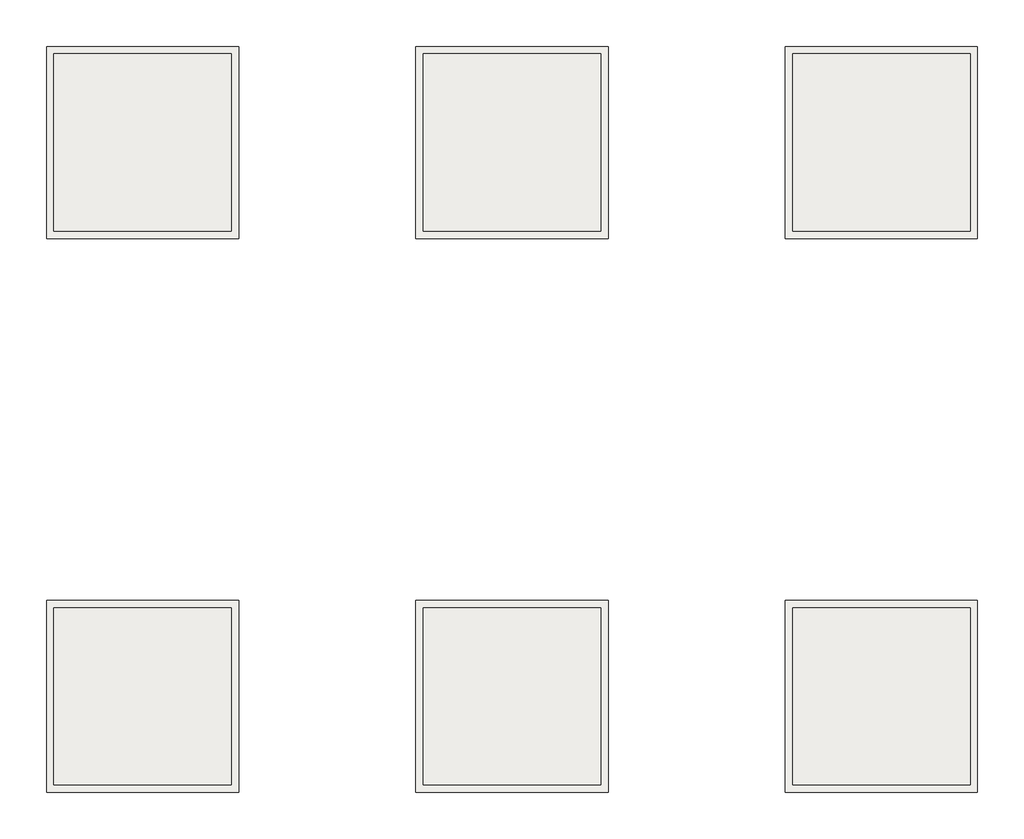
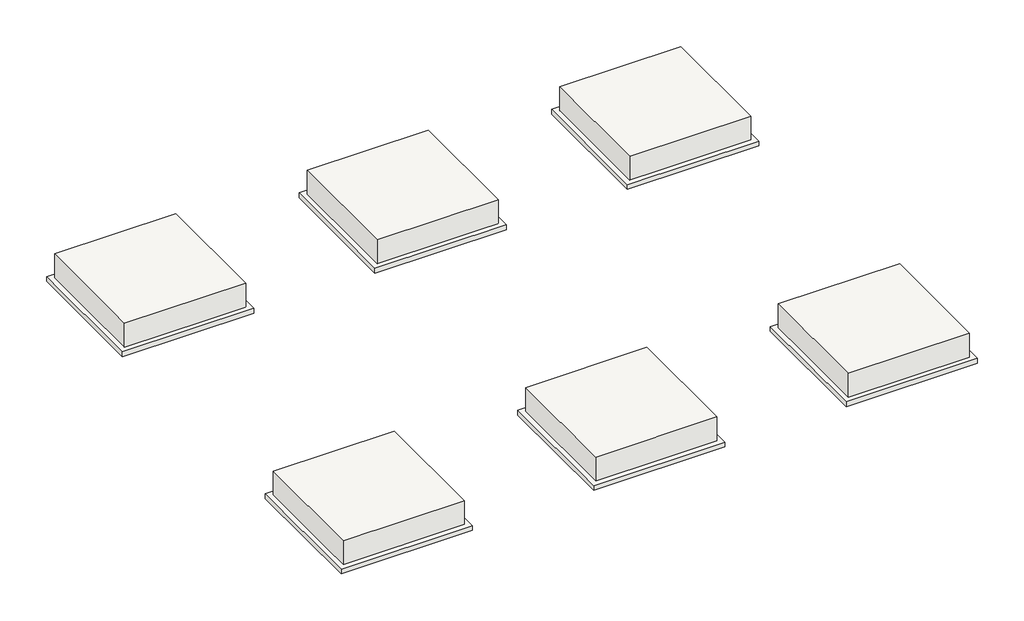
# Not in any storey: 12 slabs.
"""IFC4 building model written with IfcOpenShell, lengths in millimetres."""

import ifcopenshell
import ifcopenshell.guid

model = None  # the IFC model being written
_history = None  # IfcOwnerHistory: only IFC2X3 demands one
_inside = {}  # id of a spatial element -> (the spatial element, [elements in it])
_under = {}  # id of a project, library or spatial element -> (it, [spatial elements below it])
_declared = {}  # id of a project -> (the project, [libraries it declares])
_typed = {}  # id of a type object -> (the type object, [elements of that type])
_made_of = {}  # id of a material, layer set ... -> (it, [elements and type objects made of it])


def new_model(schema):
    """Start an empty IFC model of exactly this schema.

    Asked for "IFC4X3", IfcOpenShell would pick the latest addendum, in which some entities
    have other attributes; the version numbers below select the first issue.
    IFC2X3 requires an IfcOwnerHistory on every rooted entity: one is made here for all.
    """
    global model, _history
    if schema == "IFC4X3":
        model = ifcopenshell.file(schema_version=(4, 3, 0, 0))
    else:
        model = ifcopenshell.file(schema=schema)
    _inside.clear()
    _under.clear()
    _declared.clear()
    _typed.clear()
    _made_of.clear()
    _history = None
    if model.schema == "IFC2X3":
        org = make("IfcOrganization", Name="unknown")
        user = make(
            "IfcPersonAndOrganization",
            ThePerson=make("IfcPerson", FamilyName="unknown"),
            TheOrganization=org,
        )
        app = make(
            "IfcApplication",
            ApplicationDeveloper=org,
            Version="unknown",
            ApplicationFullName="unknown",
            ApplicationIdentifier="unknown",
        )
        _history = make(
            "IfcOwnerHistory",
            OwningUser=user,
            OwningApplication=app,
            ChangeAction="ADDED",
            CreationDate=0,
        )
    return model


def make(cls, **values):
    """One entity of the class cls with the attributes given. An attribute that is None is left unset."""
    return model.create_entity(
        cls, **{name: value for name, value in values.items() if value is not None}
    )


def rooted(cls, **values):
    """An entity with a GlobalId (a new one), such as an element, a storey or a relation."""
    return make(cls, GlobalId=ifcopenshell.guid.new(), OwnerHistory=_history, **values)


def si_unit(unit_type, name, prefix=None):
    """IfcSIUnit, for example si_unit("LENGTHUNIT", "METRE", prefix="MILLI")."""
    return make("IfcSIUnit", UnitType=unit_type, Prefix=prefix, Name=name)


def assignment(units):
    """IfcUnitAssignment: the units of a project."""
    return None if units is None else make("IfcUnitAssignment", Units=units)


def point(xyz):
    """IfcCartesianPoint."""
    return None if xyz is None else make("IfcCartesianPoint", Coordinates=xyz)


def direction(xyz):
    """IfcDirection."""
    return None if xyz is None else make("IfcDirection", DirectionRatios=xyz)


def frame(location, z_axis=None, x_axis=None):
    """IfcAxis2Placement3D, a coordinate frame: its origin and axes. An axis left out is left unset."""
    return make(
        "IfcAxis2Placement3D",
        Location=point(location),
        Axis=direction(z_axis),
        RefDirection=direction(x_axis),
    )


def origin():
    """The frame at (0, 0, 0) with its axes left unset."""
    return frame((0.0, 0.0, 0.0))


def place(relative_to, where):
    """IfcLocalPlacement: puts the frame where relative to a parent placement (None: the world)."""
    return make(
        "IfcLocalPlacement", PlacementRelTo=relative_to, RelativePlacement=where
    )


def context(
    kind, dimensions, precision=None, world=None, true_north=None, identifier=None
):
    """IfcGeometricRepresentationContext, for example the 3D "Model" context."""
    return make(
        "IfcGeometricRepresentationContext",
        ContextIdentifier=identifier,
        ContextType=kind,
        CoordinateSpaceDimension=dimensions,
        Precision=precision,
        WorldCoordinateSystem=world,
        TrueNorth=true_north,
    )


def project(units=None, contexts=None):
    """IfcProject with its units and contexts."""
    return rooted(
        "IfcProject",
        Name="project",
        RepresentationContexts=contexts,
        UnitsInContext=assignment(units),
    )


def spatial(cls, under=None, at=None, **own):
    """A site, building, storey or space (cls), placed at a placement, below another one or the project."""
    s = rooted(cls, ObjectPlacement=at, **own)
    if under is not None:
        _under.setdefault(under.id(), (under, []))[1].append(s)
    return s


def polyline(points):
    """IfcPolyline through the points."""
    return make("IfcPolyline", Points=[point(p) for p in points])


def outline(outer, holes=None, kind="AREA"):
    """IfcArbitraryClosedProfileDef: a profile drawn as a closed curve; with holes, ...WithVoids."""
    if holes is None:
        return make("IfcArbitraryClosedProfileDef", ProfileType=kind, OuterCurve=outer)
    return make(
        "IfcArbitraryProfileDefWithVoids",
        ProfileType=kind,
        OuterCurve=outer,
        InnerCurves=holes,
    )


def extrude(swept, where, along, depth):
    """IfcExtrudedAreaSolid: the profile swept, set in the frame where, extruded along a direction by depth."""
    return make(
        "IfcExtrudedAreaSolid",
        SweptArea=swept,
        Position=where,
        ExtrudedDirection=direction(along),
        Depth=depth,
    )


def shape(context_of_items, identifier, shape_type, items):
    """IfcShapeRepresentation: the items that make up one representation, for example the "Body"."""
    return make(
        "IfcShapeRepresentation",
        ContextOfItems=context_of_items,
        RepresentationIdentifier=identifier,
        RepresentationType=shape_type,
        Items=items,
    )


def made_of(thing, what):
    """Note that an element or type object is made of a material, layer set ...; save() writes the relation."""
    if what is not None:
        _made_of.setdefault(what.id(), (what, []))[1].append(thing)
    return thing


def element(
    cls,
    number,
    at=None,
    inside=None,
    cuts=None,
    type_object=None,
    material=None,
    context=None,
    identifier="Body",
    shape_type=None,
    held_by="IfcProductDefinitionShape",
    body=None,
    shapes=None,
    **own,
):
    """One element of the class cls, such as IfcWall. Its Tag is "e" and its number.

    at: its placement. inside: the storey or other place that contains it. cuts: it is an
    opening in that element (IfcRelVoidsElement). A single representation is given by context,
    identifier, shape_type and body (its items); several are given by shapes. held_by: the class
    of the entity that holds the representations. save() writes the other relations.
    """
    e = rooted(cls, Tag="e%d" % number, ObjectPlacement=at, **own)
    if body is not None:
        shapes = [shape(context, identifier, shape_type, body)]
    if shapes is not None:
        e.Representation = make(held_by, Representations=shapes)
    if inside is not None:
        _inside.setdefault(inside.id(), (inside, []))[1].append(e)
    if cuts is not None:
        rooted(
            "IfcRelVoidsElement", RelatingBuildingElement=cuts, RelatedOpeningElement=e
        )
    if type_object is not None:
        _typed.setdefault(type_object.id(), (type_object, []))[1].append(e)
    return made_of(e, material)


def aggregate(whole, parts):
    """IfcRelAggregates: a whole, such as a stair, and the parts it consists of."""
    return rooted("IfcRelAggregates", RelatingObject=whole, RelatedObjects=parts)


def save(model, path):
    """Write the relations noted so far, then the file.

    IfcRelAggregates (storeys below a building ...), IfcRelContainedInSpatialStructure (elements
    in a storey), IfcRelDefinesByType, IfcRelAssociatesMaterial and IfcRelDeclares: one each for
    every whole, place, type object, material and project.
    """
    for whole, parts in _under.values():
        aggregate(whole, parts)
    for where, things in _inside.values():
        rooted(
            "IfcRelContainedInSpatialStructure",
            RelatedElements=things,
            RelatingStructure=where,
        )
    for kind, things in _typed.values():
        rooted("IfcRelDefinesByType", RelatedObjects=things, RelatingType=kind)
    for what, things in _made_of.values():
        rooted("IfcRelAssociatesMaterial", RelatedObjects=things, RelatingMaterial=what)
    for by, libraries in _declared.values():
        rooted("IfcRelDeclares", RelatingContext=by, RelatedDefinitions=libraries)
    model.write(path)


model = new_model("IFC4")

# Units and contexts
model_context = context("Model", 3, world=origin())
ifc_project = project(units=[si_unit("LENGTHUNIT", "METRE", prefix="MILLI")], contexts=[model_context])

# Site, building
site = spatial("IfcSite", under=ifc_project)
building = spatial("IfcBuilding", under=site)

# Slabs
placement = place(None, origin())
element("IfcSlab", 1, ObjectType="H_SF_ACF_Lean_T100", at=placement, inside=building, context=model_context, shape_type="SweptSolid", body=[
    extrude(outline(polyline([(-1300.0, 22299.5208589), (1300.0, 22299.5208589), (1300.0, 19699.5208589), (-1300.0, 19699.5208589), (-1300.0, 22299.5208589)])), frame((0.0, 0.0, -1600.0), z_axis=(0.0, 0.0, 1.0), x_axis=(1.0, 0.0, 0.0)), (0.0, 0.0, 1.0), 100.0),
])
element("IfcSlab", 2, ObjectType="H_SF_ACF_Lean_T100", at=placement, inside=building, context=model_context, shape_type="SweptSolid", body=[
    extrude(outline(polyline([(-1300.0, 14799.5208589), (1300.0, 14799.5208589), (1300.0, 12199.5208589), (-1300.0, 12199.5208589), (-1300.0, 14799.5208589)])), frame((0.0, 0.0, -1600.0), z_axis=(0.0, 0.0, 1.0), x_axis=(1.0, 0.0, 0.0)), (0.0, 0.0, 1.0), 100.0),
])
element("IfcSlab", 3, ObjectType="H_SF_ACF_Lean_T100", at=placement, inside=building, context=model_context, shape_type="SweptSolid", body=[
    extrude(outline(polyline([(3700.0, 22299.5208589), (6300.0, 22299.5208589), (6300.0, 19699.5208589), (3700.0, 19699.5208589), (3700.0, 22299.5208589)])), frame((0.0, 0.0, -1600.0), z_axis=(0.0, 0.0, 1.0), x_axis=(1.0, 0.0, 0.0)), (0.0, 0.0, 1.0), 100.0),
])
element("IfcSlab", 4, ObjectType="H_SF_ACF_Lean_T100", at=placement, inside=building, context=model_context, shape_type="SweptSolid", body=[
    extrude(outline(polyline([(3700.0, 14799.5208589), (6300.0, 14799.5208589), (6300.0, 12199.5208589), (3700.0, 12199.5208589), (3700.0, 14799.5208589)])), frame((0.0, 0.0, -1600.0), z_axis=(0.0, 0.0, 1.0), x_axis=(1.0, 0.0, 0.0)), (0.0, 0.0, 1.0), 100.0),
])
element("IfcSlab", 5, ObjectType="H_SF_ACF_Lean_T100", at=placement, inside=building, context=model_context, shape_type="SweptSolid", body=[
    extrude(outline(polyline([(8700.0, 22299.5208589), (11300.0, 22299.5208589), (11300.0, 19699.5208589), (8700.0, 19699.5208589), (8700.0, 22299.5208589)])), frame((0.0, 0.0, -1600.0), z_axis=(0.0, 0.0, 1.0), x_axis=(1.0, 0.0, 0.0)), (0.0, 0.0, 1.0), 100.0),
])
element("IfcSlab", 6, ObjectType="H_SF_ACF_Lean_T100", at=placement, inside=building, context=model_context, shape_type="SweptSolid", body=[
    extrude(outline(polyline([(8700.0, 14799.5208589), (11300.0, 14799.5208589), (11300.0, 12199.5208589), (8700.0, 12199.5208589), (8700.0, 14799.5208589)])), frame((0.0, 0.0, -1600.0), z_axis=(0.0, 0.0, 1.0), x_axis=(1.0, 0.0, 0.0)), (0.0, 0.0, 1.0), 100.0),
])
element("IfcSlab", 7, ObjectType="Foundation Rectangular (Non-Pile) : H_SF_ACF_W2400xL2400xT500", at=placement, inside=building, context=model_context, shape_type="SweptSolid", body=[
    extrude(outline(polyline([(6200.0, 14699.5208589), (6200.0, 12299.5208589), (3800.0, 12299.5208589), (3800.0, 14699.5208589), (6200.0, 14699.5208589)])), frame((0.0, 0.0, -1500.0), z_axis=(0.0, 0.0, 1.0), x_axis=(1.0, 0.0, 0.0)), (0.0, 0.0, 1.0), 500.0),
])
element("IfcSlab", 8, ObjectType="Foundation Rectangular (Non-Pile) : H_SF_ACF_W2400xL2400xT500", at=placement, inside=building, context=model_context, shape_type="SweptSolid", body=[
    extrude(outline(polyline([(11200.0, 14699.5208589), (11200.0, 12299.5208589), (8800.0, 12299.5208589), (8800.0, 14699.5208589), (11200.0, 14699.5208589)])), frame((0.0, 0.0, -1500.0), z_axis=(0.0, 0.0, 1.0), x_axis=(1.0, 0.0, 0.0)), (0.0, 0.0, 1.0), 500.0),
])
element("IfcSlab", 9, ObjectType="Foundation Rectangular (Non-Pile) : H_SF_ACF_W2400xL2400xT500", at=placement, inside=building, context=model_context, shape_type="SweptSolid", body=[
    extrude(outline(polyline([(11200.0, 22199.5208589), (11200.0, 19799.5208589), (8800.0, 19799.5208589), (8800.0, 22199.5208589), (11200.0, 22199.5208589)])), frame((0.0, 0.0, -1500.0), z_axis=(0.0, 0.0, 1.0), x_axis=(1.0, 0.0, 0.0)), (0.0, 0.0, 1.0), 500.0),
])
element("IfcSlab", 10, ObjectType="Foundation Rectangular (Non-Pile) : H_SF_ACF_W2400xL2400xT500", at=placement, inside=building, context=model_context, shape_type="SweptSolid", body=[
    extrude(outline(polyline([(6200.0, 22199.5208589), (6200.0, 19799.5208589), (3800.0, 19799.5208589), (3800.0, 22199.5208589), (6200.0, 22199.5208589)])), frame((0.0, 0.0, -1500.0), z_axis=(0.0, 0.0, 1.0), x_axis=(1.0, 0.0, 0.0)), (0.0, 0.0, 1.0), 500.0),
])
element("IfcSlab", 11, ObjectType="Foundation Rectangular (Non-Pile) : H_SF_ACF_W2400xL2400xT500", at=placement, inside=building, context=model_context, shape_type="SweptSolid", body=[
    extrude(outline(polyline([(1200.0, 22199.5208589), (1200.0, 19799.5208589), (-1200.0, 19799.5208589), (-1200.0, 22199.5208589), (1200.0, 22199.5208589)])), frame((0.0, 0.0, -1500.0), z_axis=(0.0, 0.0, 1.0), x_axis=(1.0, 0.0, 0.0)), (0.0, 0.0, 1.0), 500.0),
])
element("IfcSlab", 12, ObjectType="Foundation Rectangular (Non-Pile) : H_SF_ACF_W2400xL2400xT500", at=placement, inside=building, context=model_context, shape_type="SweptSolid", body=[
    extrude(outline(polyline([(1200.0, 14699.5208589), (1200.0, 12299.5208589), (-1200.0, 12299.5208589), (-1200.0, 14699.5208589), (1200.0, 14699.5208589)])), frame((0.0, 0.0, -1500.0), z_axis=(0.0, 0.0, 1.0), x_axis=(1.0, 0.0, 0.0)), (0.0, 0.0, 1.0), 500.0),
])

save(model, "model.ifc")

# Revit data of these elements
# Project information
#   Building Name = "MAIN GATE SECURITY BUILDING"
#   Project Status = "Project Status"
#   Client Name = "현대엔지니어링"
#   Project Address = "서울시 종로구 율곡로 75(계동)"
#   Project Name = "Therma Visayas Energy Project"
#   Project Number = "-"
#   BuildingbookInternationalBuildNumber = "ZgA=BAAAAA==2023BgFlAAAAAQoAAAABAQAAAAYBZAAAAAHnBwAABAQAAAABWwIAAAcH0"
# Grids (mm)
#   "A": line (0, 24502.793) -> (0, 11308.625)
#   "B": line (5000, 24502.793) -> (5000, 11308.625)
#   "C": line (10000, 24502.793) -> (10000, 11308.625)
#   "1": line (-3860.098, 13499.521) -> (12441.468, 13499.521)
#   "2": line (-3860.098, 20999.521) -> (12441.468, 20999.521)
# Type "H_SF_ACF_Lean_T100"
#   Type Comments = "구조_콘크리트"
#   Layers, outside or top first: 0.0000 m "A04AR138-00003_Hardener Finish(Powder Type)" (function 100); 0.1000 m "A03AC034-00004_Lean Concrete (including Form work)" (function 1); 0.0000 m "A03AC035-00001_Form Work (3 times in use)_Flat" (function 100); 0.0000 m "A01ZZ012-00001_PE Sheet (Vapor Barrier)_Earth" (function 100)
# Type "Foundation Rectangular (Non-Pile) : H_SF_ACF_W2400xL2400xT500"
#   Top bar = "D25@300"
#   Description = "UG Shallow Foundation"
#   Bottom bar = "D20@300"
#   Width = 2.4000 m
#   Length = 2.4000 m
#   Foundation Thickness = 0.5000 m
#   Structural Material [instance default] = A03AC032-00007_Structural Concrete_Type1_25MPa-30Mpa
#   Assembly Code = ""
# Elements 1, 2, 3, 4, 5, 6 (IfcSlab, "H_SF_ACF_Lean_T100")
#   Comments = ""
#   Height Offset From Level = 0.0000 m
#   built-in parameter 1001954 = 1
#   Phase Created = New Construction
#   Materials on its faces: "A01ZZ012-00001_PE Sheet (Vapor Barrier)_Earth", "A04AR138-00003_Hardener Finish(Powder Type)"
# Elements 7, 8, 9, 10, 11, 12 (IfcSlab, "Foundation Rectangular (Non-Pile) : H_SF_ACF_W2400xL2400xT500")
#   Comments = ""
#   Mark = "F1"
#   Structural Material = A03AC032-00007_Structural Concrete_Type1_25MPa-30Mpa
#   Phase Created = New Construction
#   Materials on its faces: "A03AC032-00007_Structural Concrete_Type1_25MPa-30Mpa"
# Materials
#   "A04AR138-00003_Hardener Finish(Powder Type)": class "Finish", colour RGB 176 176 176, transparency 0, Description = "Hardner", Cost = 0
#   "A03AC034-00004_Lean Concrete (including Form work)": class "Concrete", colour RGB 176 176 176, transparency 0, Description = "Plain Conc.", Cost = 0
#   "A03AC035-00001_Form Work (3 times in use)_Flat": class "Wood", colour RGB 149 120 74, transparency 0, Description = "Plywood", Cost = 0
#   "A01ZZ012-00001_PE Sheet (Vapor Barrier)_Earth": class "Finish", colour RGB 128 128 64, transparency 0, Description = "Plastic", Cost = 0
#   "A03AC032-00007_Structural Concrete_Type1_25MPa-30Mpa": class "Concrete", colour RGB 176 176 176, transparency 0, Keynote = "09910.A1", Description = "Reinf. Conc.", Cost = 0
